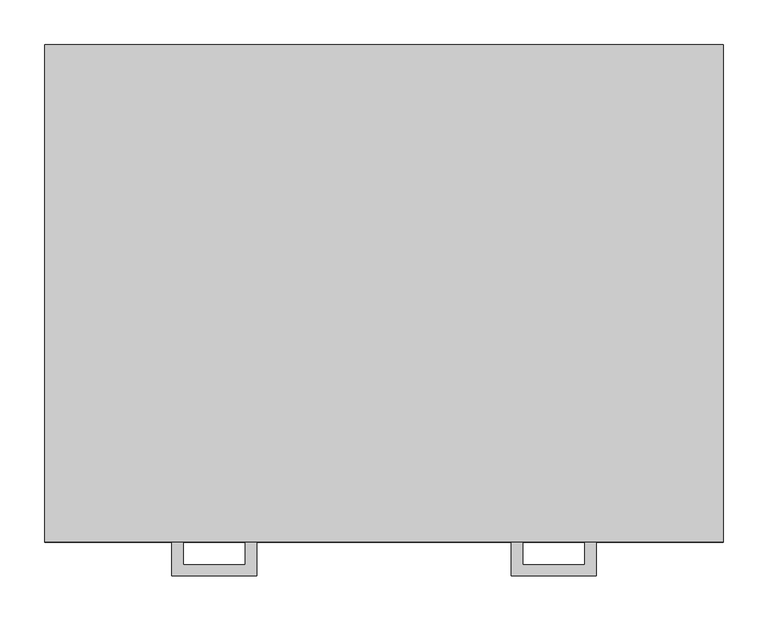
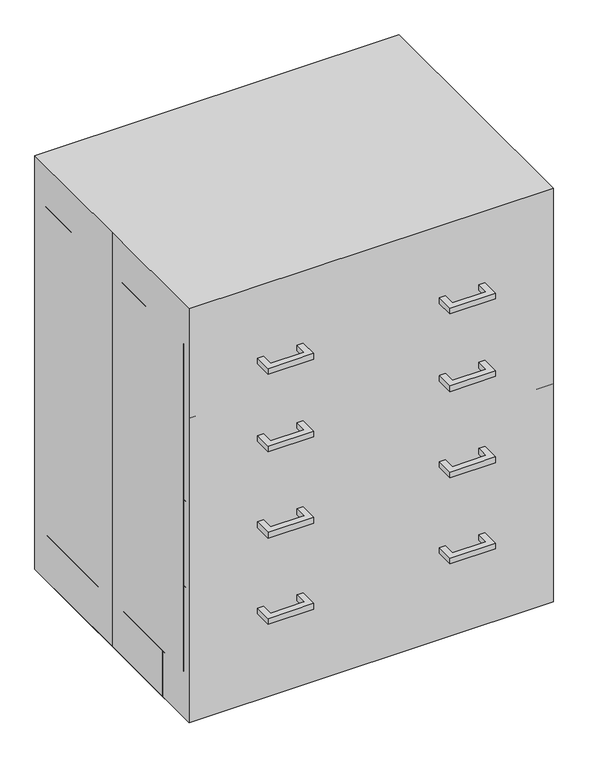
"""IFC4 building model written with IfcOpenShell, lengths in millimetres: proxy geometry, C03J0 - Cabinet, U-C-B, 8 Half DR, 36x30x22 : C03J0 - Cabinet, U-C-B, 8 Half DR, 36x30x22."""

from ifc_helpers import new_model, si_unit, frame, origin, origin_with_axes, place, context, project, spatial, polyline, outline, extrude, source, transform, mapped, element, save


def specialty_equipment_975b04b3(model_context):
    return source(origin(), model_context, "Body", "SweptSolid", [
        extrude(outline(polyline([(-238.125, -317.5), (-238.125, -279.4), (-225.4409299, -279.4), (-225.4409299, -304.8159299), (-155.5590701, -304.8159299), (-155.5590701, -279.4), (-142.875, -279.4), (-142.875, -317.5), (-238.125, -317.5)])), frame((0.0, 0.0, 571.451215), z_axis=(0.0, 0.0, 1.0), x_axis=(1.0, 0.0, 0.0)), (0.0, 0.0, 1.0), 12.7),
        extrude(outline(polyline([(238.125, -317.5), (142.875, -317.5), (142.875, -279.4), (155.5590701, -279.4), (155.5590701, -304.8159299), (225.4409299, -304.8159299), (225.4409299, -279.4), (238.125, -279.4), (238.125, -317.5)])), frame((0.0, 0.0, 571.451215), z_axis=(0.0, 0.0, 1.0), x_axis=(1.0, 0.0, 0.0)), (0.0, 0.0, 1.0), 12.7),
        extrude(outline(polyline([(-238.125, -317.5), (-238.125, -279.4), (-225.4409299, -279.4), (-225.4409299, -304.8159299), (-155.5590701, -304.8159299), (-155.5590701, -279.4), (-142.875, -279.4), (-142.875, -317.5), (-238.125, -317.5)])), frame((0.0, 0.0, 380.951215), z_axis=(0.0, 0.0, 1.0), x_axis=(1.0, 0.0, 0.0)), (0.0, 0.0, 1.0), 12.7),
        extrude(outline(polyline([(238.125, -317.5), (142.875, -317.5), (142.875, -279.4), (155.5590701, -279.4), (155.5590701, -304.8159299), (225.4409299, -304.8159299), (225.4409299, -279.4), (238.125, -279.4), (238.125, -317.5)])), frame((0.0, 0.0, 380.951215), z_axis=(0.0, 0.0, 1.0), x_axis=(1.0, 0.0, 0.0)), (0.0, 0.0, 1.0), 12.7),
        extrude(outline(polyline([(-238.125, -317.5), (-238.125, -279.4), (-225.4409299, -279.4), (-225.4409299, -304.8159299), (-155.5590701, -304.8159299), (-155.5590701, -279.4), (-142.875, -279.4), (-142.875, -317.5), (-238.125, -317.5)])), frame((0.0, 0.0, 190.4837383), z_axis=(0.0, 0.0, 1.0), x_axis=(1.0, 0.0, 0.0)), (0.0, 0.0, 1.0), 12.7),
        extrude(outline(polyline([(238.125, -317.5), (142.875, -317.5), (142.875, -279.4), (155.5590701, -279.4), (155.5590701, -304.8159299), (225.4409299, -304.8159299), (225.4409299, -279.4), (238.125, -279.4), (238.125, -317.5)])), frame((0.0, 0.0, 190.4837383), z_axis=(0.0, 0.0, 1.0), x_axis=(1.0, 0.0, 0.0)), (0.0, 0.0, 1.0), 12.7),
        extrude(outline(polyline([(-238.125, -317.5), (-238.125, -279.4), (-225.4409299, -279.4), (-225.4409299, -304.8159299), (-155.5590701, -304.8159299), (-155.5590701, -279.4), (-142.875, -279.4), (-142.875, -317.5), (-238.125, -317.5)])), frame((0.0, 0.0, 742.9174767), z_axis=(0.0, 0.0, 1.0), x_axis=(1.0, 0.0, 0.0)), (0.0, 0.0, 1.0), 12.7),
        extrude(outline(polyline([(238.125, -317.5), (142.875, -317.5), (142.875, -279.4), (155.5590701, -279.4), (155.5590701, -304.8159299), (225.4409299, -304.8159299), (225.4409299, -279.4), (238.125, -279.4), (238.125, -317.5)])), frame((0.0, 0.0, 742.9174767), z_axis=(0.0, 0.0, 1.0), x_axis=(1.0, 0.0, 0.0)), (0.0, 0.0, 1.0), 12.7),
        extrude(outline(polyline([(-381.0, 279.4), (381.0, 279.4), (381.0, -279.4), (-381.0, -279.4), (-381.0, 0.0), (-381.0, 279.4)])), origin_with_axes(), (0.0, 0.0, 1.0), 914.4),
        extrude(outline(polyline([(381.0, -279.4), (0.0, -279.4), (0.0, -260.35), (381.0, -260.35), (381.0, -279.4)])), frame((0.0, 0.0, 101.6), z_axis=(0.0, 0.0, 1.0), x_axis=(1.0, 0.0, 0.0)), (0.0, 0.0, 1.0), 190.4674767),
        extrude(outline(polyline([(0.0, -279.4), (-381.0, -279.4), (-381.0, -260.35), (0.0, -260.35), (0.0, -279.4)])), frame((0.0, 0.0, 101.6), z_axis=(0.0, 0.0, 1.0), x_axis=(1.0, 0.0, 0.0)), (0.0, 0.0, 1.0), 190.4674767),
        extrude(outline(polyline([(381.0, -279.4), (0.0, -279.4), (0.0, -260.35), (381.0, -260.35), (381.0, -279.4)])), frame((0.0, 0.0, 292.0674767), z_axis=(0.0, 0.0, 1.0), x_axis=(1.0, 0.0, 0.0)), (0.0, 0.0, 1.0), 190.5),
        extrude(outline(polyline([(0.0, -279.4), (-381.0, -279.4), (-381.0, -260.35), (0.0, -260.35), (0.0, -279.4)])), frame((0.0, 0.0, 292.0674767), z_axis=(0.0, 0.0, 1.0), x_axis=(1.0, 0.0, 0.0)), (0.0, 0.0, 1.0), 190.5),
        extrude(outline(polyline([(381.0, -279.4), (0.0, -279.4), (0.0, -260.35), (381.0, -260.35), (381.0, -279.4)])), frame((0.0, 0.0, 482.5674767), z_axis=(0.0, 0.0, 1.0), x_axis=(1.0, 0.0, 0.0)), (0.0, 0.0, 1.0), 190.5),
        extrude(outline(polyline([(0.0, -279.4), (-381.0, -279.4), (-381.0, -260.35), (0.0, -260.35), (0.0, -279.4)])), frame((0.0, 0.0, 482.5674767), z_axis=(0.0, 0.0, 1.0), x_axis=(1.0, 0.0, 0.0)), (0.0, 0.0, 1.0), 190.5),
        extrude(outline(polyline([(381.0, -279.4), (0.0, -279.4), (0.0, -260.35), (381.0, -260.35), (381.0, -279.4)])), frame((0.0, 0.0, 673.0674767), z_axis=(0.0, 0.0, 1.0), x_axis=(1.0, 0.0, 0.0)), (0.0, 0.0, 1.0), 152.4),
        extrude(outline(polyline([(0.0, -279.4), (-381.0, -279.4), (-381.0, -260.35), (0.0, -260.35), (0.0, -279.4)])), frame((0.0, 0.0, 673.0674767), z_axis=(0.0, 0.0, 1.0), x_axis=(1.0, 0.0, 0.0)), (0.0, 0.0, 1.0), 152.4),
        extrude(outline(polyline([(-381.0, -260.35), (-381.0, 279.4), (-361.95, 279.4), (-361.95, -260.35), (-381.0, -260.35)])), frame((0.0, 0.0, 101.6), z_axis=(0.0, 0.0, 1.0), x_axis=(1.0, 0.0, 0.0)), (0.0, 0.0, 1.0), 723.8674767),
        extrude(outline(polyline([(361.95, -260.35), (361.95, 279.4), (381.0, 279.4), (381.0, -260.35), (361.95, -260.35)])), frame((0.0, 0.0, 101.6), z_axis=(0.0, 0.0, 1.0), x_axis=(1.0, 0.0, 0.0)), (0.0, 0.0, 1.0), 723.8674767),
        extrude(outline(polyline([(381.0, -203.2), (-381.0, -203.2), (-381.0, -184.15), (381.0, -184.15), (381.0, -203.2)])), origin_with_axes(), (0.0, 0.0, 1.0), 101.6),
        extrude(outline(polyline([(-381.0, -184.15), (-381.0, 279.4), (-361.95, 279.4), (-361.95, -184.15), (-381.0, -184.15)])), origin_with_axes(), (0.0, 0.0, 1.0), 101.6),
        extrude(outline(polyline([(361.95, -184.15), (361.95, 279.4), (381.0, 279.4), (381.0, -184.15), (361.95, -184.15)])), origin_with_axes(), (0.0, 0.0, 1.0), 101.6),
        extrude(outline(polyline([(381.0, 260.35), (-381.0, 260.35), (-381.0, 279.4), (381.0, 279.4), (381.0, 260.35)])), origin_with_axes(), (0.0, 0.0, 1.0), 101.6),
        extrude(outline(polyline([(361.95, 260.35), (361.95, -260.35), (-361.95, -260.35), (-361.95, 260.35), (361.95, 260.35)])), frame((0.0, 0.0, 101.6), z_axis=(0.0, 0.0, 1.0), x_axis=(1.0, 0.0, 0.0)), (0.0, 0.0, 1.0), 19.1166954),
        extrude(outline(polyline([(361.95, 260.35), (-361.95, 260.35), (-361.95, 279.4), (361.95, 279.4), (361.95, 260.35)])), frame((0.0, 0.0, 101.6), z_axis=(0.0, 0.0, 1.0), x_axis=(1.0, 0.0, 0.0)), (0.0, 0.0, 1.0), 704.8174767),
    ])


if __name__ == "__main__":
    model = new_model("IFC4")
    model_context = context("Model", 3, world=origin())
    ifc_project = project(units=[si_unit("LENGTHUNIT", "METRE", prefix="MILLI")], contexts=[model_context])
    site = spatial("IfcSite", under=ifc_project)
    building = spatial("IfcBuilding", under=site)
    placement = place(None, origin())
    specialty_equipment_shape = specialty_equipment_975b04b3(model_context)
    element("IfcBuildingElementProxy", 1, Name="C03J0 - Cabinet, U-C-B, 8 Half DR, 36x30x22 : C03J0 - Cabinet, U-C-B, 8 Half DR, 36x30x22", ObjectType="C03J0 - Cabinet, U-C-B, 8 Half DR, 36x30x22 : C03J0 - Cabinet, U-C-B, 8 Half DR, 36x30x22", at=placement, inside=building, context=model_context, shape_type="MappedRepresentation", body=[
        mapped(specialty_equipment_shape, transform((0.0, 0.0, 0.0), x_axis=(1.0, 0.0, 0.0), y_axis=(0.0, 1.0, 0.0), z_axis=(0.0, 0.0, 1.0))),
    ])
    save(model, "model.ifc")

# Revit data of these elements
# Type "C03J0 - Cabinet, U-C-B, 8 Half DR, 36x30x22 : C03J0 - Cabinet, U-C-B, 8 Half DR, 36x30x22"
#   Watts2 = "0"
#   Watts1 = "0"
#   Unit_Issue = "EA"
#   UTIL_6_Misc = "-"
#   UTIL_5_NonMedGas = "-"
#   UTIL_4_MiscGas = "-"
#   UTIL_3_MedGas = "-"
#   UTIL_2_Elec = "-"
#   UTIL_1_WaterDrain = "-"
#   Nomenclature = "Cabinet, U/C/B, 8 Half Drawers, 36x30x22"
#   NSN = "6530"
#   Location [instance default] = ""
#   JSN = "C03J0"
#   Fund_Source_VA = "-"
#   Fund_Source_Navy = "-"
#   Fund_Source_Army = "-"
#   Fund_Source_AF = "-"
#   ELEC_Volts2 = "0"
#   ELEC_Volts1 = "0"
#   ELEC_Phase2 = "0"
#   ELEC_Phase1 = "0"
#   ELEC_HertzSwitch = "0"
#   ELEC_HertzDependent = "0"
#   ELEC_Hertz = "0"
#   ELEC_Amps2 = "0"
#   ELEC_Amps1 = "0"
#   DetailDescription = "Standing height under counter base cabinet with two half width drawers side-by-side above three full width drawers. Also referred to as a drawer cabinet. For general purpose use throughout the facility."
#   CAT_VA = "A"
#   CAT_Navy = "A"
#   CAT_IHS = "-"
#   CAT_Army = "A"
#   CAT_AF = "A"
#   BTUperhour = "0"
#   Weight_IP = 150
#   DIM_Width_IP = 2' - 6"
#   DIM_Height_IP = 3' - 0"
#   DIM_Depth_IP = 1' - 10"
#   Top Panel Material = none
#   Toe Panel Material = none
#   Side Panel Material = none
#   Shelf Panel Material = none
#   Drawer Front Material = none
#   Door Panel Material = none
#   Back Panel Material = none
#   Assembly Code = ""
# Element 1 (IfcBuildingElementProxy, "C03J0 - Cabinet, U-C-B, 8 Half DR, 36x30x22 : C03J0 - Cabinet, U-C-B, 8 Half DR, 36x30x22")
#   Materials on its faces: "Default metal", "EquipSpace"
# Materials
#   "Default metal": class "Unassigned", colour RGB 204 204 204, transparency 0
#   "EquipSpace": class "Unassigned", colour RGB 221 217 195, transparency 0.5
